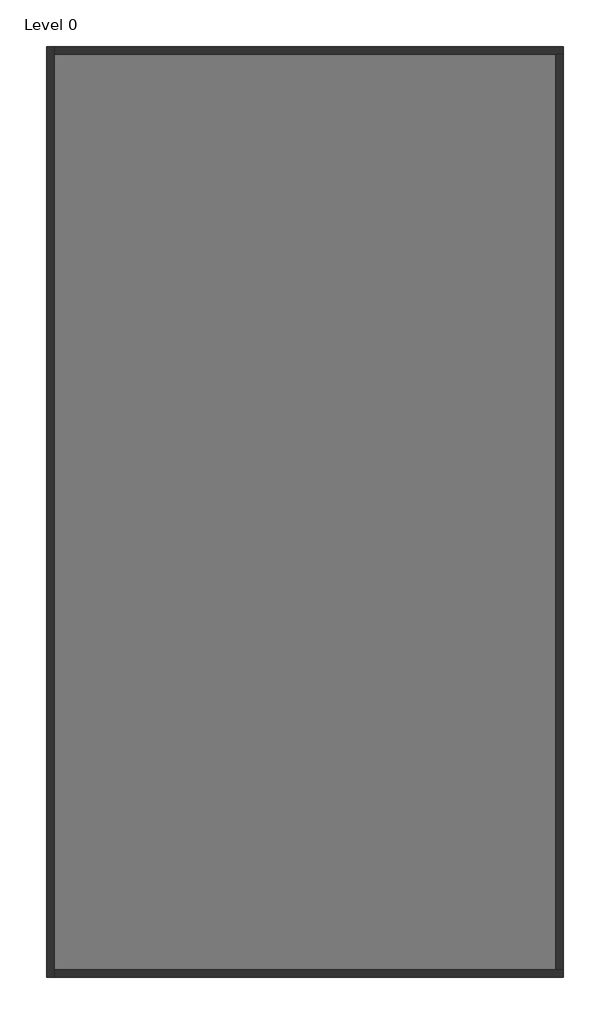
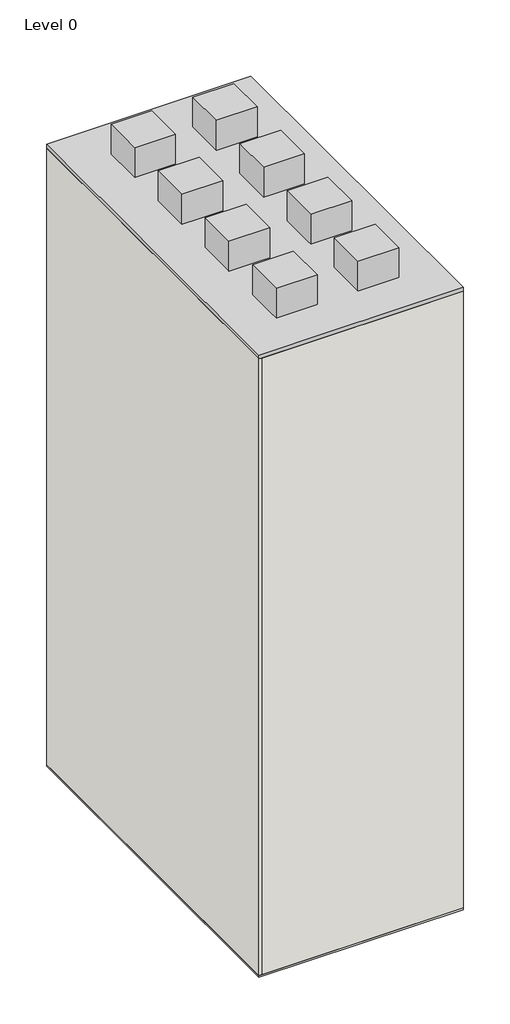
# One storey: 4 walls, 1 proxy, 1 slab.
"""IFC4 building model written with IfcOpenShell, lengths in millimetres."""

from ifc_helpers import new_model, si_unit, frame, origin, origin_with_axes, place, context, project, spatial, polyline, outline, extrude, faceted_brep, element, save

model = new_model("IFC4")

# Units and contexts
model_context = context("Model", 3, world=origin())
ifc_project = project(units=[si_unit("LENGTHUNIT", "METRE", prefix="MILLI")], contexts=[model_context])

# Site, building, storey
site = spatial("IfcSite", under=ifc_project)
building = spatial("IfcBuilding", under=site)
storey = spatial("IfcBuildingStorey", under=building, Name="Level 0", Elevation=100.0)

# Proxy
placement = place(None, origin())
element("IfcBuildingElementProxy", 1, Name="LowUrbanDensityBuilding : LowUrbanDensityBuilding", ObjectType="LowUrbanDensityBuilding : LowUrbanDensityBuilding", at=placement, inside=storey, context=model_context, shape_type="SweptSolid", body=[
    extrude(outline(polyline([(7325.2659446, 3676.2074539), (7325.2659446, -14323.7925461), (-2674.7340554, -14323.7925461), (-2674.7340554, 3676.2074539), (7325.2659446, 3676.2074539)])), origin_with_axes(), (0.0, 0.0, 1.0), 32200.0),
    extrude(outline(polyline([(1325.2659446, 1676.2074539), (1325.2659446, -323.7925461), (-674.7340554, -323.7925461), (-674.7340554, 1676.2074539), (1325.2659446, 1676.2074539)])), frame((0.0, 0.0, 32000.0), z_axis=(0.0, 0.0, 1.0), x_axis=(1.0, 0.0, 0.0)), (0.0, 0.0, 1.0), 1749.8),
    extrude(outline(polyline([(5325.2659446, 1676.2074539), (5325.2659446, -323.7925461), (3325.2659446, -323.7925461), (3325.2659446, 1676.2074539), (5325.2659446, 1676.2074539)])), frame((0.0, 0.0, 32000.0), z_axis=(0.0, 0.0, 1.0), x_axis=(1.0, 0.0, 0.0)), (0.0, 0.0, 1.0), 1749.8),
    extrude(outline(polyline([(1325.2659446, -2323.7925461), (1325.2659446, -4323.7925461), (-674.7340554, -4323.7925461), (-674.7340554, -2323.7925461), (1325.2659446, -2323.7925461)])), frame((0.0, 0.0, 32000.0), z_axis=(0.0, 0.0, 1.0), x_axis=(1.0, 0.0, 0.0)), (0.0, 0.0, 1.0), 1749.8),
    extrude(outline(polyline([(5325.2659446, -2323.7925461), (5325.2659446, -4323.7925461), (3325.2659446, -4323.7925461), (3325.2659446, -2323.7925461), (5325.2659446, -2323.7925461)])), frame((0.0, 0.0, 32000.0), z_axis=(0.0, 0.0, 1.0), x_axis=(1.0, 0.0, 0.0)), (0.0, 0.0, 1.0), 1749.8),
    extrude(outline(polyline([(1325.2659446, -6323.7925461), (1325.2659446, -8323.7925461), (-674.7340554, -8323.7925461), (-674.7340554, -6323.7925461), (1325.2659446, -6323.7925461)])), frame((0.0, 0.0, 32000.0), z_axis=(0.0, 0.0, 1.0), x_axis=(1.0, 0.0, 0.0)), (0.0, 0.0, 1.0), 1749.8),
    extrude(outline(polyline([(5325.2659446, -6323.7925461), (5325.2659446, -8323.7925461), (3325.2659446, -8323.7925461), (3325.2659446, -6323.7925461), (5325.2659446, -6323.7925461)])), frame((0.0, 0.0, 32000.0), z_axis=(0.0, 0.0, 1.0), x_axis=(1.0, 0.0, 0.0)), (0.0, 0.0, 1.0), 1749.8),
    extrude(outline(polyline([(1325.2659446, -10323.7925461), (1325.2659446, -12323.7925461), (-674.7340554, -12323.7925461), (-674.7340554, -10323.7925461), (1325.2659446, -10323.7925461)])), frame((0.0, 0.0, 32000.0), z_axis=(0.0, 0.0, 1.0), x_axis=(1.0, 0.0, 0.0)), (0.0, 0.0, 1.0), 1749.8),
    extrude(outline(polyline([(5325.2659446, -10323.7925461), (5325.2659446, -12323.7925461), (3325.2659446, -12323.7925461), (3325.2659446, -10323.7925461), (5325.2659446, -10323.7925461)])), frame((0.0, 0.0, 32000.0), z_axis=(0.0, 0.0, 1.0), x_axis=(1.0, 0.0, 0.0)), (0.0, 0.0, 1.0), 1749.8),
])

# Slab
element("IfcSlab", 2, ObjectType="Floor-Concrete_100Con", at=placement, inside=storey, context=model_context, shape_type="SweptSolid", body=[
    extrude(outline(polyline([(7325.2659446, 3676.2074539), (7325.2659446, -14323.7925461), (-2674.7340554, -14323.7925461), (-2674.7340554, 3676.2074539), (7325.2659446, 3676.2074539)])), origin_with_axes(), (0.0, 0.0, 1.0), 100.0),
])

# Walls
element("IfcWall", 3, ObjectType="Wall-Ext_25Rdr-100Blk-19P", at=placement, inside=storey, context=model_context, shape_type="Brep", body=[
    faceted_brep([(-2674.7340554, 3676.2074539, 100.0), (-2674.7340554, -14323.7925461, 100.0), (-2674.7340554, -14323.7925461, 32000.0), (-2674.7340554, 3676.2074539, 32000.0), (-2530.4340554, 3676.2074539, 100.0), (-2530.4340554, 3676.2074539, 32000.0), (-2530.4340554, 3531.9074539, 32000.0), (-2530.4340554, -14179.4925461, 32000.0), (-2530.4340554, -14323.7925461, 32000.0), (-2530.4340554, -14323.7925461, 100.0), (-2530.4340554, -14179.4925461, 100.0), (-2530.4340554, 3531.9074539, 100.0)], [[[0, 1, 2, 3]], [[4, 5, 6, 7, 8, 9, 10, 11]], [[1, 0, 4, 11, 10, 9]], [[3, 2, 8, 7, 6, 5]], [[2, 1, 9, 8]], [[0, 3, 5, 4]]]),
])
element("IfcWall", 4, ObjectType="Wall-Ext_25Rdr-100Blk-19P", at=placement, inside=storey, context=model_context, shape_type="Brep", body=[
    faceted_brep([(-2530.4340554, -14323.7925461, 100.0), (7325.2659446, -14323.7925461, 100.0), (7325.2659446, -14323.7925461, 32000.0), (-2530.4340554, -14323.7925461, 32000.0), (-2530.4340554, -14179.4925461, 100.0), (-2530.4340554, -14179.4925461, 32000.0), (7180.9659446, -14179.4925461, 32000.0), (7325.2659446, -14179.4925461, 32000.0), (7325.2659446, -14179.4925461, 100.0), (7180.9659446, -14179.4925461, 100.0)], [[[0, 1, 2, 3]], [[4, 5, 6, 7, 8, 9]], [[1, 0, 4, 9, 8]], [[3, 2, 7, 6, 5]], [[0, 3, 5, 4]], [[2, 1, 8, 7]]]),
])
element("IfcWall", 5, ObjectType="Wall-Ext_25Rdr-100Blk-19P", at=placement, inside=storey, context=model_context, shape_type="Brep", body=[
    faceted_brep([(7325.2659446, 3676.2074539, 100.0), (-2530.4340554, 3676.2074539, 100.0), (-2530.4340554, 3676.2074539, 32000.0), (7325.2659446, 3676.2074539, 32000.0), (7325.2659446, 3531.9074539, 100.0), (7325.2659446, 3531.9074539, 32000.0), (7180.9659446, 3531.9074539, 32000.0), (-2530.4340554, 3531.9074539, 32000.0), (-2530.4340554, 3531.9074539, 100.0), (7180.9659446, 3531.9074539, 100.0)], [[[0, 1, 2, 3]], [[4, 5, 6, 7, 8, 9]], [[1, 0, 4, 9, 8]], [[3, 2, 7, 6, 5]], [[2, 1, 8, 7]], [[0, 3, 5, 4]]]),
])
element("IfcWall", 6, ObjectType="Wall-Ext_25Rdr-100Blk-19P", at=placement, inside=storey, context=model_context, shape_type="SweptSolid", body=[
    extrude(outline(polyline([(7325.2659446, 3531.9074539), (7325.2659446, -14179.4925461), (7180.9659446, -14179.4925461), (7180.9659446, 3531.9074539), (7325.2659446, 3531.9074539)])), frame((0.0, 0.0, 100.0), z_axis=(0.0, 0.0, 1.0), x_axis=(1.0, 0.0, 0.0)), (0.0, 0.0, 1.0), 31900.0),
])

save(model, "model.ifc")

# Revit data of these elements
# Project information
#   Project Issue Date = "Issue Date"
#   Project Status = "Project Status"
#   Client Name = "Owner"
#   Project Address = "Enter address here"
#   Project Name = "Project Name"
#   Project Number = "Project Number"
# Type "Floor-Concrete_100Con"
#   Keynote = "E60/130"
#   Function = 0
#   Layers, outside or top first: 100 mm "Concrete" (function 1)
# Type "Wall-Ext_25Rdr-100Blk-19P"
#   Keynote = "F10"
#   Layers, outside or top first: 25.3 mm "Render, Beige, Smooth" (function 5); 100 mm "Concrete Masonry Units _Low Density" (function 1); 19 mm "Plaster" (function 5)
# Element 1 (IfcBuildingElementProxy, "LowUrbanDensityBuilding : LowUrbanDensityBuilding")
#   Phase Created = New Construction
#   Materials on its faces: "Default Form"
# Element 2 (IfcSlab, "Floor-Concrete_100Con")
#   Height Offset From Level = 0 mm
#   Phase Created = New Construction
#   Materials on its faces: "Concrete"
# Element 3 (IfcWall, "Wall-Ext_25Rdr-100Blk-19P")
#   Top Offset = 0 mm
#   Base Offset = 0 mm
#   wall height = 31900 mm
#   Phase Created = New Construction
#   Base Constraint = Level 0
#   Top Constraint = Level 8
#   Materials on its faces: "Render, Beige, Smooth", "Default Wall", "Plaster"
# Elements 4, 5, 6 (IfcWall, "Wall-Ext_25Rdr-100Blk-19P")
#   Top Offset = 0 mm
#   Base Offset = 0 mm
#   wall height = 31900 mm
#   Phase Created = New Construction
#   Base Constraint = Level 0
#   Top Constraint = Level 8
#   Materials on its faces: "Default Wall", "Render, Beige, Smooth", "Plaster"
# Materials
#   "Concrete": class "Concrete", colour RGB 120 120 120, transparency 0, Description = "Portland Cement Concrete", Cost = 0
#   "Render, Beige, Smooth": class "Generic", colour RGB 213 198 180, transparency 0, Description = "physical material", Cost = 0
#   "Concrete Masonry Units _Low Density": class "Masonry", colour RGB 181 181 181, transparency 0, Description = "Concrete masonry units", Cost = 0
#   "Plaster": class "Generic", colour RGB 249 249 249, transparency 0, Description = "Plaster", Cost = 0
#   "Default Form": class "Generic", colour RGB 185 189 196, transparency 0.5, Cost = 0
#   "Default Wall": class "Miscellaneous", colour RGB 128 128 128, transparency 0, Comments = "Rendering appearance not upgraded Rendering appearance not upgraded ", Cost = 0
